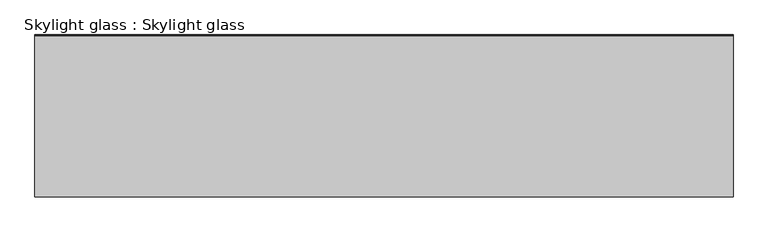
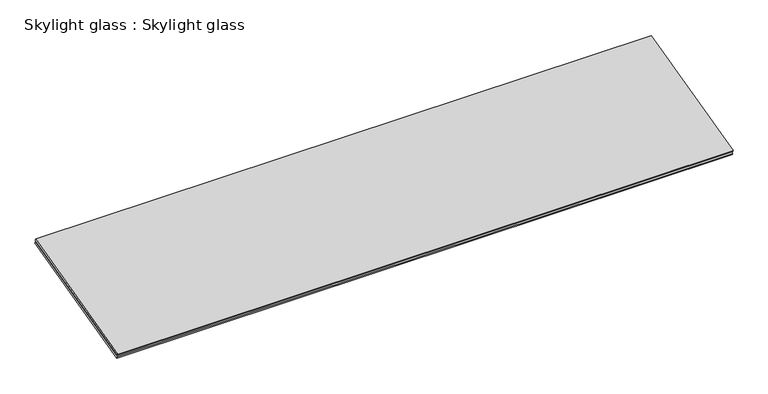
"""IFC4 building model written with IfcOpenShell, lengths in millimetres: proxy geometry, Skylight glass : Skylight glass."""

from ifc_helpers import new_model, si_unit, frame, origin, place, context, project, spatial, polyline, outline, extrude, source, transform, mapped, element, save


def skylight_glass_skylight_glass_9c3f357c(model_context):
    return source(origin(), model_context, "Body", "SweptSolid", [
        extrude(outline(polyline([(9633.4400538, 43788.1259916), (9632.3198258, 43792.6038351), (10093.7955598, 43908.0518299), (10094.9379691, 43903.4853224), (9633.4400538, 43788.1259916)])), frame((3694.2883192, 0.0, 0.0), z_axis=(1.0, 0.0, 0.0), x_axis=(0.0, 1.0, 0.0)), (0.0, 0.0, 1.0), 2000.0),
        extrude(outline(polyline([(9630.4722335, 43799.942238), (9629.3741867, 43804.3314175), (10090.8609639, 43919.782175), (10091.9811919, 43915.3043315), (9630.4722335, 43799.942238)])), frame((3694.2883192, 0.0, 0.0), z_axis=(1.0, 0.0, 0.0), x_axis=(0.0, 1.0, 0.0)), (0.0, 0.0, 1.0), 2000.0),
    ])


if __name__ == "__main__":
    model = new_model("IFC4")
    model_context = context("Model", 3, world=origin())
    ifc_project = project(units=[si_unit("LENGTHUNIT", "METRE", prefix="MILLI")], contexts=[model_context])
    site = spatial("IfcSite", under=ifc_project)
    building = spatial("IfcBuilding", under=site)
    placement = place(None, origin())
    skylight_glass_skylight_glass_shape = skylight_glass_skylight_glass_9c3f357c(model_context)
    element("IfcBuildingElementProxy", 1, Name="Skylight glass : Skylight glass", ObjectType="Skylight glass : Skylight glass", at=placement, inside=building, context=model_context, shape_type="MappedRepresentation", body=[
        mapped(skylight_glass_skylight_glass_shape, transform((0.0, 0.0, 0.0), x_axis=(1.0, 0.0, 0.0), y_axis=(0.0, 1.0, 0.0), z_axis=(0.0, 0.0, 1.0))),
    ])
    save(model, "model.ifc")

# Revit data of these elements
# Type "Skylight glass : Skylight glass"
#   NameOverride = "Skylight glass"
# Element 1 (IfcBuildingElementProxy, "Skylight glass : Skylight glass")
#   Materials on its faces: "WINDOW GLASS"
# Materials
#   "WINDOW GLASS": class "Unassigned", colour RGB 146 199 212, transparency 0
